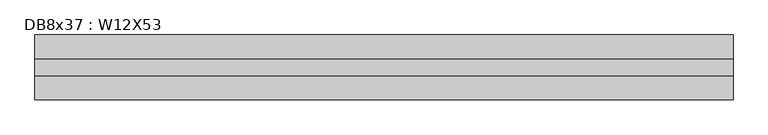
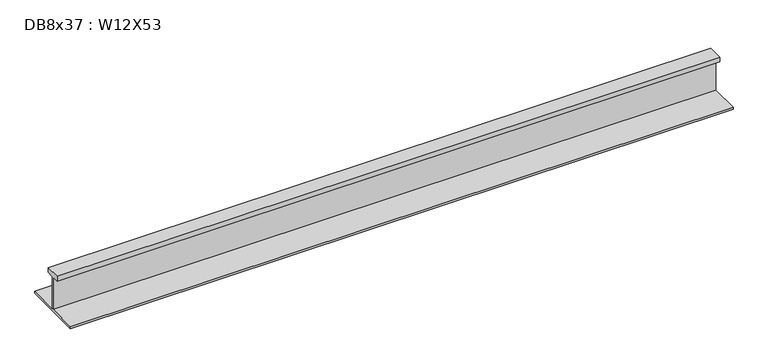
"""IFC4 building model written with IfcOpenShell, lengths in millimetres: beam geometry, DB8x37 : W12X53."""

from ifc_helpers import new_model, si_unit, frame, origin, place, context, project, spatial, polyline, outline, extrude, source, transform, mapped, element, save


def db8x37_w12x53_253518bd(model_context):
    return source(origin(), model_context, "Body", "SweptSolid", [
        extrude(outline(polyline([(38.1, 145.415), (38.1, 120.015), (2.921, 120.015), (2.921, -48.4505), (152.4, -48.4505), (152.4, -58.1025), (-152.4, -58.1025), (-152.4, -48.4505), (-2.921, -48.4505), (-2.921, 120.015), (-38.1, 120.015), (-38.1, 145.415), (38.1, 145.415)])), frame((-1612.9, 0.0, 0.0), z_axis=(1.0, 0.0, 0.0), x_axis=(0.0, 1.0, 0.0)), (0.0, 0.0, 1.0), 3276.473),
    ])


if __name__ == "__main__":
    model = new_model("IFC4")
    model_context = context("Model", 3, world=origin())
    ifc_project = project(units=[si_unit("LENGTHUNIT", "METRE", prefix="MILLI")], contexts=[model_context])
    site = spatial("IfcSite", under=ifc_project)
    building = spatial("IfcBuilding", under=site)
    placement = place(None, origin())
    db8x37_w12x53_shape = db8x37_w12x53_253518bd(model_context)
    element("IfcBeam", 1, ObjectType="DB8x37 : W12X53", at=placement, inside=building, context=model_context, shape_type="MappedRepresentation", body=[
        mapped(db8x37_w12x53_shape, transform((0.0, 0.0, 0.0), x_axis=(1.0, 0.0, 0.0), y_axis=(0.0, 1.0, 0.0), z_axis=(0.0, 0.0, 1.0))),
    ])
    save(model, "model.ifc")

# Revit data of these elements
# Type "DB8x37 : W12X53"
#   Assembly Code = "B10"
#   W = 53
#   Length [instance default] = 5' - 0"
#   bf = 0' - 10"
#   d = 1' - 0.1"
#   k = 0' - 1 3/8"
#   k2 = 0' - 0.8"
#   tf = 0' - 0.575"
#   tw = 0' - 0.345"
#   A = 0.108333 SF
#   Structural Material [instance default] = Steel ASTM A992
# Element 1 (IfcBeam, "DB8x37 : W12X53")
#   Materials on its faces: "Steel ASTM A992"
# Materials
#   "Steel ASTM A992": class "Metal", colour RGB 199 199 199, transparency 0, Description = "Structural steel 50ksi", Cost = 0
